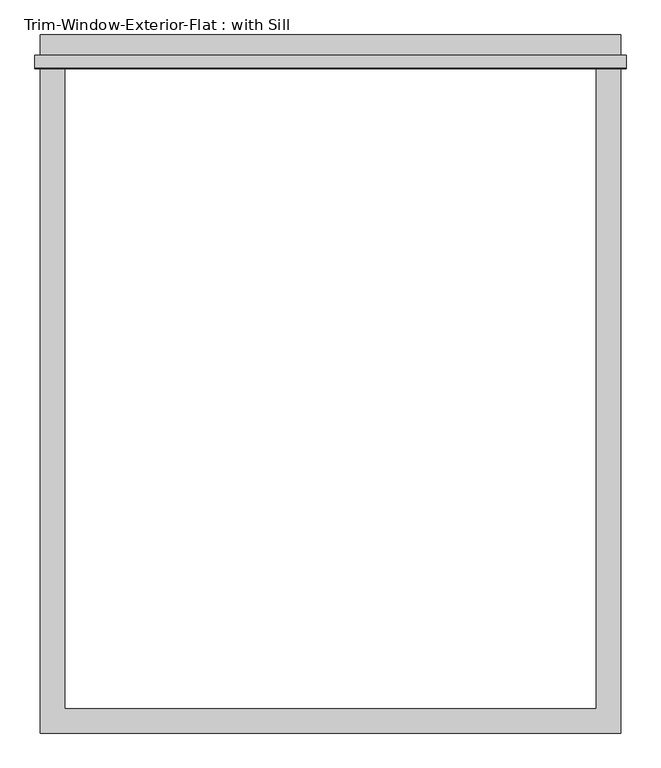
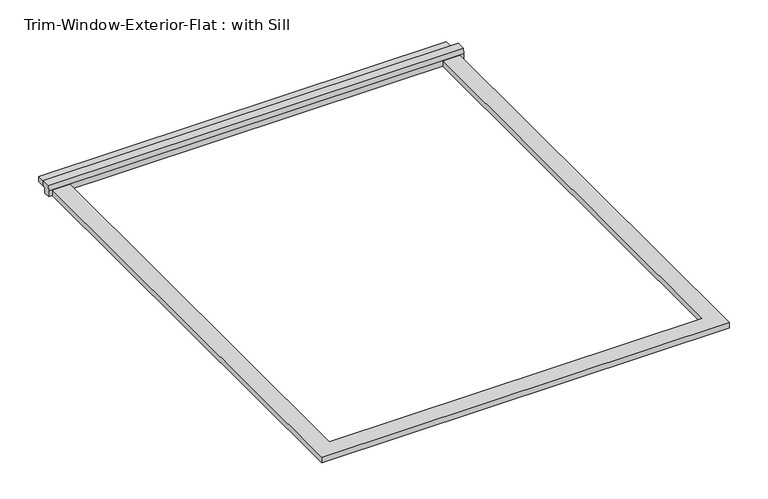
"""IFC4 building model written with IfcOpenShell, lengths in millimetres: proxy geometry, Trim-Window-Exterior-Flat : with Sill."""

from ifc_helpers import new_model, si_unit, frame, origin, origin_with_axes, place, context, project, spatial, polyline, outline, extrude, source, transform, mapped, element, save


def trim_window_exterior_flat_with_sill_9a477a0d(model_context):
    return source(origin(), model_context, "Body", "SweptSolid", [
        extrude(outline(polyline([(679.45, 1520.7823709), (-679.45, 1520.7823709), (-679.45, 1577.9323709), (679.45, 1577.9323709), (679.45, 1520.7823709)])), origin_with_axes(), (0.0, 0.0, 1.0), 19.05),
        extrude(outline(polyline([(1530.35, 38.1), (1530.35, 19.05), (1520.7823709, 19.05), (1520.7823709, 0.0), (1498.6, 0.0), (1498.6, 19.05), (1501.0580645, 38.1), (1530.35, 38.1)])), frame((-692.15, 0.0, 0.0), z_axis=(1.0, 0.0, 0.0), x_axis=(0.0, 1.0, 0.0)), (0.0, 0.0, 1.0), 1384.3),
        extrude(outline(polyline([(-679.45, -57.15), (-679.45, 1498.6), (-622.3, 1498.6), (-622.3, 0.0), (622.3, 0.0), (622.3, 1498.6), (679.45, 1498.6), (679.45, -57.15), (-679.45, -57.15)])), origin_with_axes(), (0.0, 0.0, 1.0), 19.05),
    ])


if __name__ == "__main__":
    model = new_model("IFC4")
    model_context = context("Model", 3, world=origin())
    ifc_project = project(units=[si_unit("LENGTHUNIT", "METRE", prefix="MILLI")], contexts=[model_context])
    site = spatial("IfcSite", under=ifc_project)
    building = spatial("IfcBuilding", under=site)
    placement = place(None, origin())
    trim_window_exterior_flat_with_sill_shape = trim_window_exterior_flat_with_sill_9a477a0d(model_context)
    element("IfcBuildingElementProxy", 1, Name="Trim-Window-Exterior-Flat : with Sill", ObjectType="Trim-Window-Exterior-Flat : with Sill", at=placement, inside=building, context=model_context, shape_type="MappedRepresentation", body=[
        mapped(trim_window_exterior_flat_with_sill_shape, transform((0.0, 0.0, 0.0), x_axis=(1.0, 0.0, 0.0), y_axis=(0.0, 1.0, 0.0), z_axis=(0.0, 0.0, 1.0))),
    ])
    save(model, "model.ifc")

# Revit data of these elements
# Type "Trim-Window-Exterior-Flat : with Sill"
#   Trim Width = 0' - 2 1/4"
#   Trim Thickness_Picture Frame = 0' - 1 1/4"
#   Trim Thickness_with Sill = 0' - 0 3/4"
#   Sill Thickness = 0' - 1 1/4"
#   Opening Width [instance default] = 2' - 0"
#   Opening Height [instance default] = 3' - 0"
#   Default Elevation = 4' - 0"
#   Sill = yes
#   Picture Frame = no
#   Trim Material [instance default] = none
# Element 1 (IfcBuildingElementProxy, "Trim-Window-Exterior-Flat : with Sill")
#   Opening Width = 4' - 1"
#   Opening Height = 4' - 11"
#   Trim Material = Clad - White
#   Materials on its faces: "Clad - White"
# Materials
#   "Clad - White": class "Wood", colour RGB 242 242 238, transparency 0, Cost = 0
